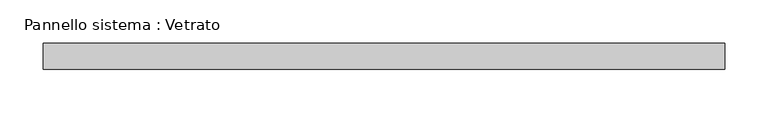
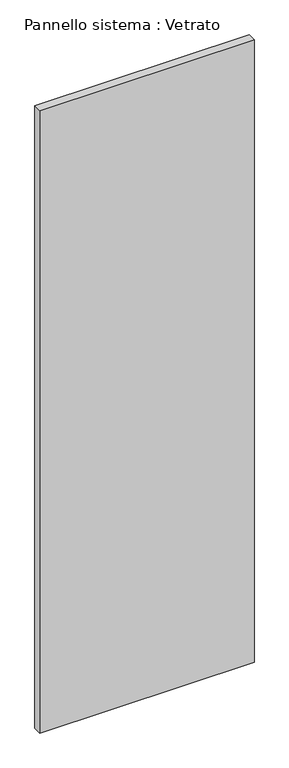
"""IFC4 building model written with IfcOpenShell, lengths in millimetres: plate geometry, Pannello sistema : Vetrato."""

from ifc_helpers import new_model, si_unit, origin, origin_with_axes, place, context, project, spatial, polyline, outline, extrude, source, transform, mapped, element, save


def pannello_sistema_vetrato_acecd054(model_context):
    return source(origin(), model_context, "Body", "SweptSolid", [
        extrude(outline(polyline([(395.0, -15.0), (-395.0, -15.0), (-395.0, 15.0), (395.0, 15.0), (395.0, -15.0)])), origin_with_axes(), (0.0, 0.0, 1.0), 2425.0),
    ])


if __name__ == "__main__":
    model = new_model("IFC4")
    model_context = context("Model", 3, world=origin())
    ifc_project = project(units=[si_unit("LENGTHUNIT", "METRE", prefix="MILLI")], contexts=[model_context])
    site = spatial("IfcSite", under=ifc_project)
    building = spatial("IfcBuilding", under=site)
    placement = place(None, origin())
    pannello_sistema_vetrato_shape = pannello_sistema_vetrato_acecd054(model_context)
    element("IfcPlate", 1, ObjectType="Pannello sistema : Vetrato", at=placement, inside=building, context=model_context, shape_type="MappedRepresentation", body=[
        mapped(pannello_sistema_vetrato_shape, transform((0.0, 0.0, 0.0), x_axis=(1.0, 0.0, 0.0), y_axis=(0.0, 1.0, 0.0), z_axis=(0.0, 0.0, 1.0))),
    ])
    save(model, "model.ifc")

# Revit data of these elements
# Type "Pannello sistema : Vetrato"
#   Construction Type Id = "GSP4R"
#   Analytic Construction = "Vetrata singola Pilkington 1/8 in"
#   Visual Light Transmittance = 0.9
#   Solar Heat Gain Coefficient = 0.86
#   Heat Transfer Coefficient (U) = 6.7069 W/(m²·K)
# Element 1 (IfcPlate, "Pannello sistema : Vetrato")
#   Materials on its faces: "Default - Vetro"
# Materials
#   "Default - Vetro": class "Vetro", colour RGB 208 208 208, transparency 0.7, Cost = 0
